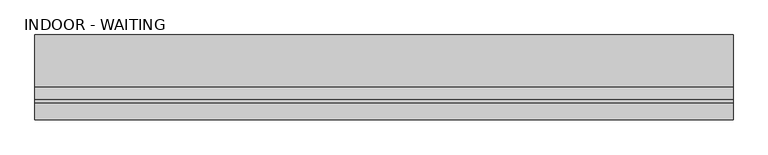
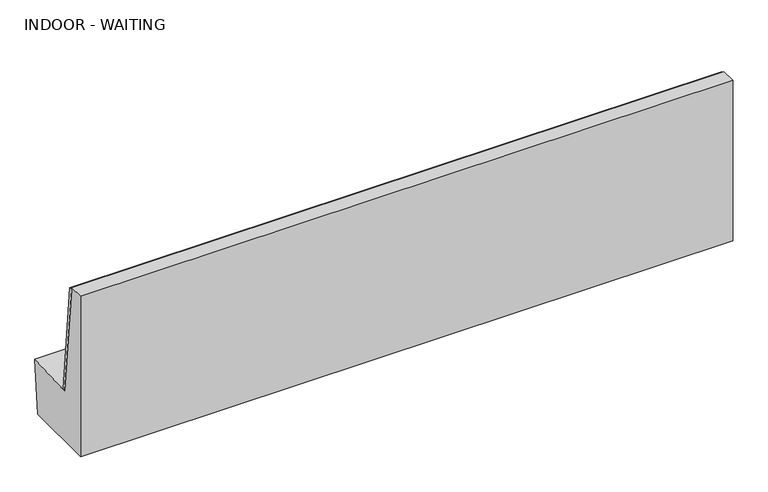
"""IFC4 building model written with IfcOpenShell, lengths in millimetres: furniture geometry, OD_CW_Booth : INDOOR - WAITING."""

from ifc_helpers import new_model, si_unit, frame, origin, place, context, project, spatial, polyline, outline, extrude, source, transform, mapped, element, save


def indoor_waiting_3751da6a(model_context):
    return source(origin(), model_context, "Body", "SweptSolid", [
        extrude(outline(polyline([(0.0, -5377.2445204), (0.0, 0.0), (25.4, 0.0), (25.4, -5377.2445204), (0.0, -5377.2445204)])), frame((5395.9822253, -358.2049359, 438.8309433), z_axis=(0.0, -0.10452846326765197, 0.9945218953682735), x_axis=(0.0, -0.9945218953682735, -0.10452846326765197)), (0.0, 0.0, 1.0), 944.7333479),
        extrude(outline(polyline([(-609.6, 1397.0), (-484.4524721, 1397.0), (-382.9385128, 431.1591941), (43.0849153, 453.4861359), (3.4100193, 0.0), (-609.6, 0.0), (-609.6, 1397.0)])), frame((18.7377049, 0.0, 0.0), z_axis=(1.0, 0.0, 0.0), x_axis=(0.0, 1.0, 0.0)), (0.0, 0.0, 1.0), 5377.2445204),
    ])


if __name__ == "__main__":
    model = new_model("IFC4")
    model_context = context("Model", 3, world=origin())
    ifc_project = project(units=[si_unit("LENGTHUNIT", "METRE", prefix="MILLI")], contexts=[model_context])
    site = spatial("IfcSite", under=ifc_project)
    building = spatial("IfcBuilding", under=site)
    placement = place(None, origin())
    indoor_waiting_shape = indoor_waiting_3751da6a(model_context)
    element("IfcFurniture", 1, ObjectType="OD_CW_Booth : INDOOR - WAITING", at=placement, inside=building, context=model_context, shape_type="MappedRepresentation", body=[
        mapped(indoor_waiting_shape, transform((0.0, 0.0, 0.0), x_axis=(1.0, 0.0, 0.0), y_axis=(0.0, 1.0, 0.0), z_axis=(0.0, 0.0, 1.0))),
    ])
    save(model, "model.ifc")

# Revit data of these elements
# Type "OD_CW_Booth : INDOOR - WAITING"
#   Width = 4' - 0"
#   OD_CW_Width [instance default] = 2' - 10"
#   OD_CW_Length [instance default] = 26' - 1 83/256"
#   OD_CW_Height [instance default] = 2' - 3"
#   Height = 3' - 0"
#   Depth = 2' - 0"
#   Seating Count [instance default] = 10
#   back = WOOD VENEER
#   OD_CW_Material_Front Panel [instance default] = none
#   OD_CW_Material_Body [instance default] = none
# Element 1 (IfcFurniture, "OD_CW_Booth : INDOOR - WAITING")
#   OD_CW_Length = 17' - 7.70254"
#   Seating Count = 7
#   OD_CW_Material_Body = WOOD-OAKFIRE
#   Materials on its faces: "WOOD-OAKFIRE", "WOOD VENEER"
# Materials
#   "WOOD VENEER": class "Miscellaneous", colour RGB 164 164 164, transparency 0, Cost = 0
#   "WOOD-OAKFIRE": class "Wood", colour RGB 198 202 183, transparency 0, Description = "Generic wood", Cost = 0
